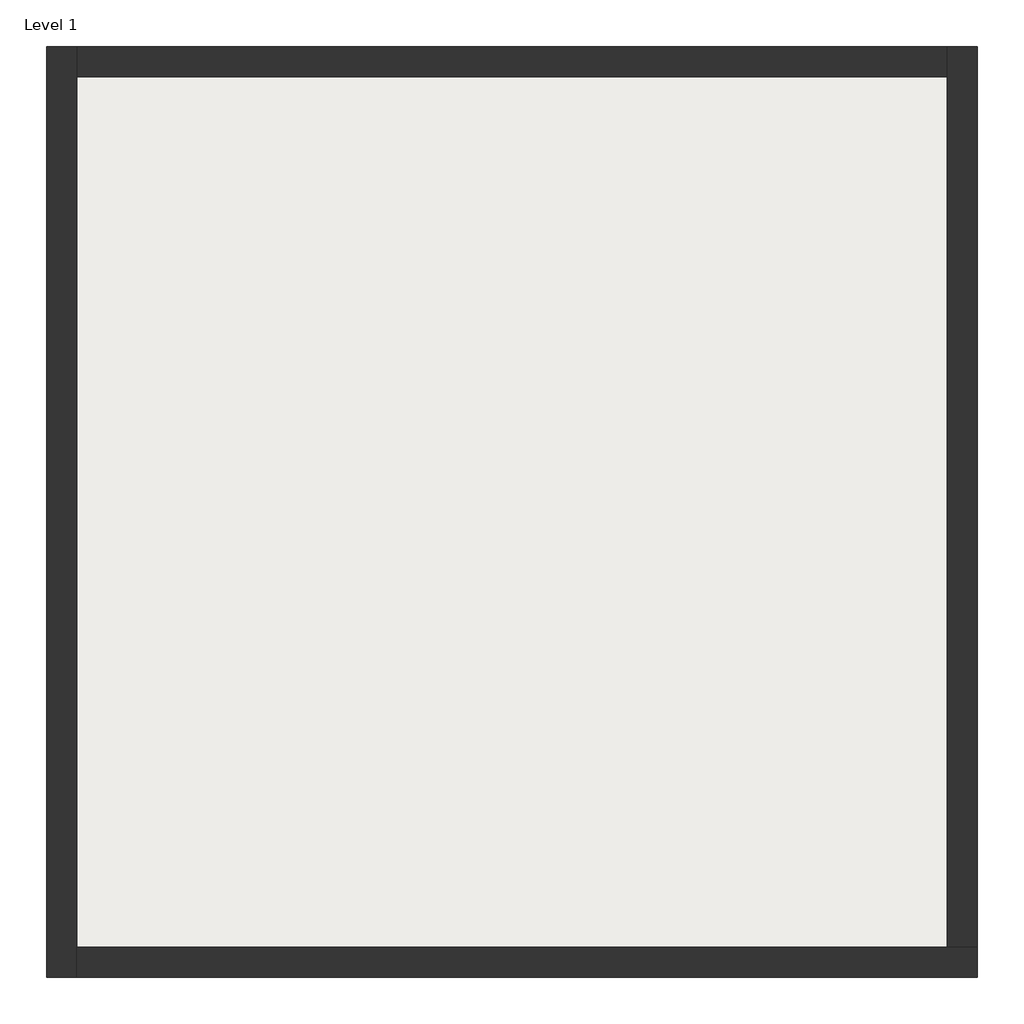
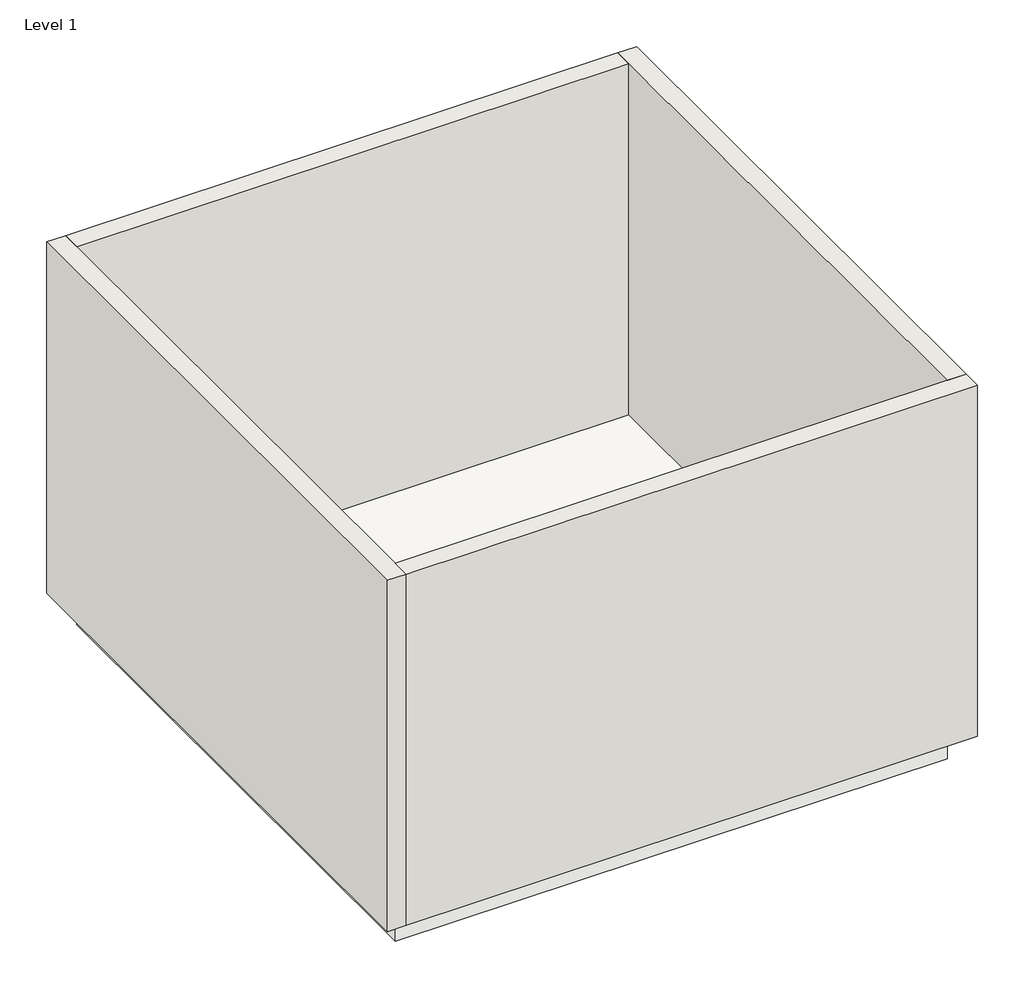
# One storey: 4 walls, 1 slab.
"""IFC4 building model written with IfcOpenShell, lengths in millimetres."""

from ifc_helpers import new_model, si_unit, frame, origin, origin_with_axes, place, context, project, spatial, polyline, outline, extrude, faceted_brep, element, save

model = new_model("IFC4")

# Units and contexts
model_context = context("Model", 3, world=origin())
ifc_project = project(units=[si_unit("LENGTHUNIT", "METRE", prefix="MILLI")], contexts=[model_context])

# Site, building, storey
site = spatial("IfcSite", under=ifc_project)
building = spatial("IfcBuilding", under=site)
storey = spatial("IfcBuildingStorey", under=building, Name="Level 1", Elevation=0.0)

# Slab
placement = place(None, origin())
element("IfcSlab", 1, ObjectType="Generic - 12\"", at=placement, inside=storey, context=model_context, shape_type="SweptSolid", body=[
    extrude(outline(polyline([(-11616.6724061, 8921.0385252), (-5723.8724061, 8921.0385252), (-5723.8724061, 3028.2385252), (-11616.6724061, 3028.2385252), (-11616.6724061, 8921.0385252)])), frame((0.0, 0.0, -304.8), z_axis=(0.0, 0.0, 1.0), x_axis=(1.0, 0.0, 0.0)), (0.0, 0.0, 1.0), 304.8),
])

# Walls
element("IfcWall", 2, ObjectType="Generic - 8\"", at=placement, inside=storey, context=model_context, shape_type="Brep", body=[
    faceted_brep([(-11819.8724061, 9124.2385252, 0.0), (-11819.8724061, 2825.0385252, 0.0), (-11819.8724061, 2825.0385252, 3962.4), (-11819.8724061, 9124.2385252, 3962.4), (-11616.6724061, 9124.2385252, 0.0), (-11616.6724061, 9124.2385252, 3962.4), (-11616.6724061, 8921.0385252, 3962.4), (-11616.6724061, 3028.2385252, 3962.4), (-11616.6724061, 2825.0385252, 3962.4), (-11616.6724061, 2825.0385252, 0.0), (-11616.6724061, 3028.2385252, 0.0), (-11616.6724061, 8921.0385252, 0.0)], [[[0, 1, 2, 3]], [[4, 5, 6, 7, 8, 9, 10, 11]], [[1, 0, 4, 11, 10, 9]], [[3, 2, 8, 7, 6, 5]], [[2, 1, 9, 8]], [[0, 3, 5, 4]]]),
])
element("IfcWall", 3, ObjectType="Generic - 8\"", at=placement, inside=storey, context=model_context, shape_type="Brep", body=[
    faceted_brep([(-11616.6724061, 2825.0385252, 0.0), (-5520.6724061, 2825.0385252, 0.0), (-5520.6724061, 2825.0385252, 3962.4), (-11616.6724061, 2825.0385252, 3962.4), (-11616.6724061, 3028.2385252, 0.0), (-11616.6724061, 3028.2385252, 3962.4), (-5723.8724061, 3028.2385252, 3962.4), (-5520.6724061, 3028.2385252, 3962.4), (-5520.6724061, 3028.2385252, 0.0), (-5723.8724061, 3028.2385252, 0.0)], [[[0, 1, 2, 3]], [[4, 5, 6, 7, 8, 9]], [[1, 0, 4, 9, 8]], [[3, 2, 7, 6, 5]], [[0, 3, 5, 4]], [[2, 1, 8, 7]]]),
])
element("IfcWall", 4, ObjectType="Generic - 8\"", at=placement, inside=storey, context=model_context, shape_type="Brep", body=[
    faceted_brep([(-5520.6724061, 3028.2385252, 0.0), (-5520.6724061, 9124.2385252, 0.0), (-5520.6724061, 9124.2385252, 3962.4), (-5520.6724061, 3028.2385252, 3962.4), (-5723.8724061, 3028.2385252, 0.0), (-5723.8724061, 3028.2385252, 3962.4), (-5723.8724061, 8921.0385252, 3962.4), (-5723.8724061, 9124.2385252, 3962.4), (-5723.8724061, 9124.2385252, 0.0), (-5723.8724061, 8921.0385252, 0.0)], [[[0, 1, 2, 3]], [[4, 5, 6, 7, 8, 9]], [[1, 0, 4, 9, 8]], [[3, 2, 7, 6, 5]], [[0, 3, 5, 4]], [[2, 1, 8, 7]]]),
])
element("IfcWall", 5, ObjectType="Generic - 8\"", at=placement, inside=storey, context=model_context, shape_type="SweptSolid", body=[
    extrude(outline(polyline([(-11616.6724061, 9124.2385252), (-5723.8724061, 9124.2385252), (-5723.8724061, 8921.0385252), (-11616.6724061, 8921.0385252), (-11616.6724061, 9124.2385252)])), origin_with_axes(), (0.0, 0.0, 1.0), 3962.4),
])

save(model, "model.ifc")

# Revit data of these elements
# Project information
#   Project Issue Date = "Issue Date"
#   Project Status = "Project Status"
#   Client Name = "Owner"
#   Project Address = "Enter address here"
#   Project Name = "Project Name"
#   Project Number = "Project Number"
# Type "Generic - 12\""
#   Assembly Code = "B1010"
#   Function = 0
#   Layers, outside or top first: 1' - 0" no material (function 1)
# Type "Generic - 8\""
#   Assembly Code = "B2010"
#   Layers, outside or top first: 0' - 8" no material (function 1)
# Element 1 (IfcSlab, "Generic - 12\"")
#   built-in parameter 1001955 = 3.14159 (stored number, unit not read)
#   Height Offset From Level = 0' - 0"
#   Phase Created = New Construction
#   Materials on its faces: "Default Floor"
# Elements 2, 3, 4, 5 (IfcWall, "Generic - 8\"")
#   Top Offset = 0' - 0"
#   Base Offset = 0' - 0"
#   wall height = 13' - 0"
#   Phase Created = New Construction
#   Base Constraint = Level 1
#   Top Constraint = Level 2
#   Materials on its faces: "Default Wall"
# Materials
#   "Default Floor": class "Miscellaneous", colour RGB 128 128 128, transparency 0, Cost = 0
#   "Default Wall": class "Miscellaneous", colour RGB 128 128 128, transparency 0, Cost = 0
